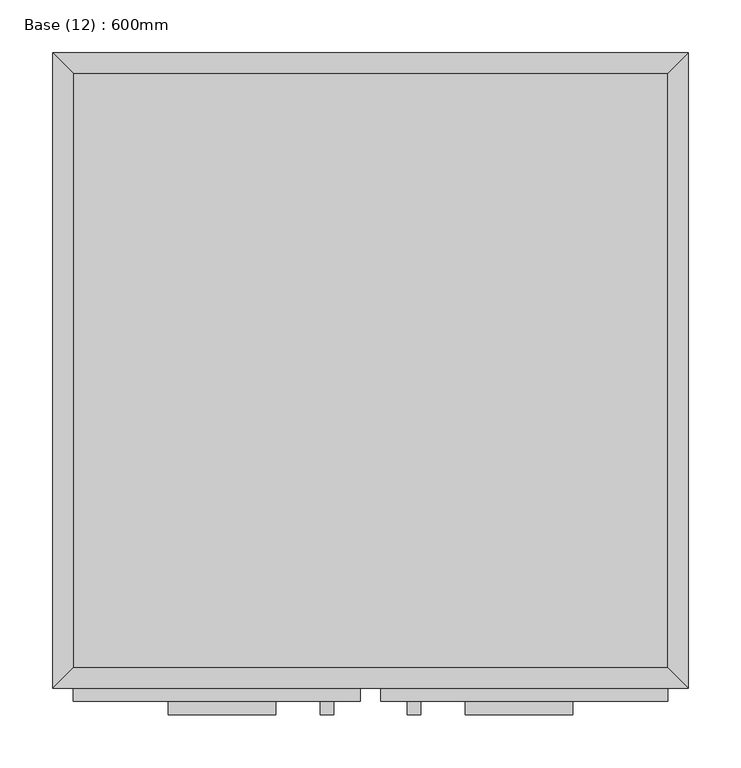
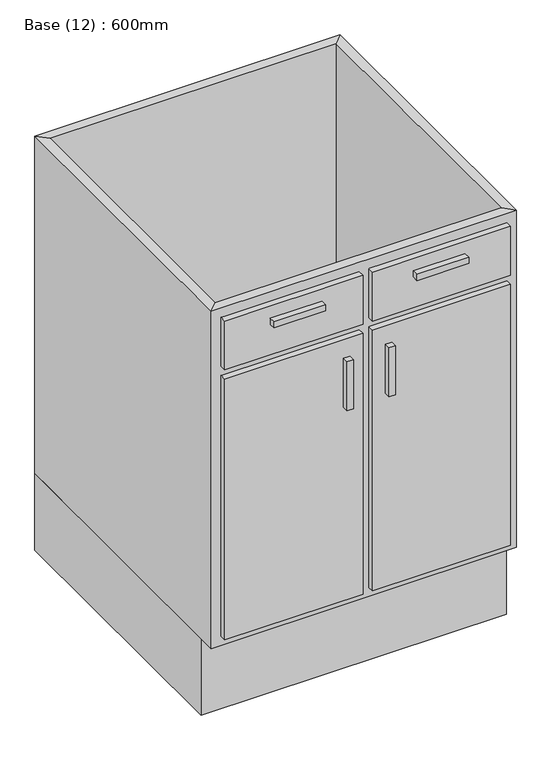
"""IFC4 building model written with IfcOpenShell, lengths in millimetres: furniture geometry, Base (12) : 600mm."""

import ifcopenshell
import ifcopenshell.guid

model = None  # the IFC model being written
_history = None  # IfcOwnerHistory: only IFC2X3 demands one
_inside = {}  # id of a spatial element -> (the spatial element, [elements in it])
_under = {}  # id of a project, library or spatial element -> (it, [spatial elements below it])
_declared = {}  # id of a project -> (the project, [libraries it declares])
_typed = {}  # id of a type object -> (the type object, [elements of that type])
_made_of = {}  # id of a material, layer set ... -> (it, [elements and type objects made of it])


def new_model(schema):
    """Start an empty IFC model of exactly this schema.

    Asked for "IFC4X3", IfcOpenShell would pick the latest addendum, in which some entities
    have other attributes; the version numbers below select the first issue.
    IFC2X3 requires an IfcOwnerHistory on every rooted entity: one is made here for all.
    """
    global model, _history
    if schema == "IFC4X3":
        model = ifcopenshell.file(schema_version=(4, 3, 0, 0))
    else:
        model = ifcopenshell.file(schema=schema)
    _inside.clear()
    _under.clear()
    _declared.clear()
    _typed.clear()
    _made_of.clear()
    _history = None
    if model.schema == "IFC2X3":
        org = make("IfcOrganization", Name="unknown")
        user = make(
            "IfcPersonAndOrganization",
            ThePerson=make("IfcPerson", FamilyName="unknown"),
            TheOrganization=org,
        )
        app = make(
            "IfcApplication",
            ApplicationDeveloper=org,
            Version="unknown",
            ApplicationFullName="unknown",
            ApplicationIdentifier="unknown",
        )
        _history = make(
            "IfcOwnerHistory",
            OwningUser=user,
            OwningApplication=app,
            ChangeAction="ADDED",
            CreationDate=0,
        )
    return model


def make(cls, **values):
    """One entity of the class cls with the attributes given. An attribute that is None is left unset."""
    return model.create_entity(
        cls, **{name: value for name, value in values.items() if value is not None}
    )


def rooted(cls, **values):
    """An entity with a GlobalId (a new one), such as an element, a storey or a relation."""
    return make(cls, GlobalId=ifcopenshell.guid.new(), OwnerHistory=_history, **values)


def si_unit(unit_type, name, prefix=None):
    """IfcSIUnit, for example si_unit("LENGTHUNIT", "METRE", prefix="MILLI")."""
    return make("IfcSIUnit", UnitType=unit_type, Prefix=prefix, Name=name)


def assignment(units):
    """IfcUnitAssignment: the units of a project."""
    return None if units is None else make("IfcUnitAssignment", Units=units)


def point(xyz):
    """IfcCartesianPoint."""
    return None if xyz is None else make("IfcCartesianPoint", Coordinates=xyz)


def direction(xyz):
    """IfcDirection."""
    return None if xyz is None else make("IfcDirection", DirectionRatios=xyz)


def frame(location, z_axis=None, x_axis=None):
    """IfcAxis2Placement3D, a coordinate frame: its origin and axes. An axis left out is left unset."""
    return make(
        "IfcAxis2Placement3D",
        Location=point(location),
        Axis=direction(z_axis),
        RefDirection=direction(x_axis),
    )


def origin():
    """The frame at (0, 0, 0) with its axes left unset."""
    return frame((0.0, 0.0, 0.0))


def origin_with_axes():
    """The frame at (0, 0, 0) with the z axis (0, 0, 1) and the x axis (1, 0, 0) written out."""
    return frame((0.0, 0.0, 0.0), z_axis=(0.0, 0.0, 1.0), x_axis=(1.0, 0.0, 0.0))


def place(relative_to, where):
    """IfcLocalPlacement: puts the frame where relative to a parent placement (None: the world)."""
    return make(
        "IfcLocalPlacement", PlacementRelTo=relative_to, RelativePlacement=where
    )


def context(
    kind, dimensions, precision=None, world=None, true_north=None, identifier=None
):
    """IfcGeometricRepresentationContext, for example the 3D "Model" context."""
    return make(
        "IfcGeometricRepresentationContext",
        ContextIdentifier=identifier,
        ContextType=kind,
        CoordinateSpaceDimension=dimensions,
        Precision=precision,
        WorldCoordinateSystem=world,
        TrueNorth=true_north,
    )


def project(units=None, contexts=None):
    """IfcProject with its units and contexts."""
    return rooted(
        "IfcProject",
        Name="project",
        RepresentationContexts=contexts,
        UnitsInContext=assignment(units),
    )


def spatial(cls, under=None, at=None, **own):
    """A site, building, storey or space (cls), placed at a placement, below another one or the project."""
    s = rooted(cls, ObjectPlacement=at, **own)
    if under is not None:
        _under.setdefault(under.id(), (under, []))[1].append(s)
    return s


def polyline(points):
    """IfcPolyline through the points."""
    return make("IfcPolyline", Points=[point(p) for p in points])


def outline(outer, holes=None, kind="AREA"):
    """IfcArbitraryClosedProfileDef: a profile drawn as a closed curve; with holes, ...WithVoids."""
    if holes is None:
        return make("IfcArbitraryClosedProfileDef", ProfileType=kind, OuterCurve=outer)
    return make(
        "IfcArbitraryProfileDefWithVoids",
        ProfileType=kind,
        OuterCurve=outer,
        InnerCurves=holes,
    )


def extrude(swept, where, along, depth):
    """IfcExtrudedAreaSolid: the profile swept, set in the frame where, extruded along a direction by depth."""
    return make(
        "IfcExtrudedAreaSolid",
        SweptArea=swept,
        Position=where,
        ExtrudedDirection=direction(along),
        Depth=depth,
    )


def faces_of(points, faces, orient=None, outer=None):
    """IfcFace entities. A face is a list of loops; a loop is a list of indices into points, from 0.

    orient and outer hold one flag for each loop. By default every Orientation is true, the
    first loop of a face is its IfcFaceOuterBound and the others are IfcFaceBound.
    """
    made = []
    for i, loops in enumerate(faces):
        bounds = []
        for j, loop in enumerate(loops):
            is_outer = j == 0 if outer is None else outer[i][j]
            bounds.append(
                make(
                    "IfcFaceOuterBound" if is_outer else "IfcFaceBound",
                    Bound=make("IfcPolyLoop", Polygon=[points[k] for k in loop]),
                    Orientation=True if orient is None else orient[i][j],
                )
            )
        made.append(make("IfcFace", Bounds=bounds))
    return made


def faceted_brep(points, faces, orient=None, outer=None, voids=None):
    """IfcFacetedBrep: a solid bounded by flat faces; with voids (closed shells), ...WithVoids."""
    shared = [point(p) for p in points]
    hull = make("IfcClosedShell", CfsFaces=faces_of(shared, faces, orient, outer))
    if voids is None:
        return make("IfcFacetedBrep", Outer=hull)
    return make(
        "IfcFacetedBrepWithVoids",
        Outer=hull,
        Voids=[
            make(cls, CfsFaces=faces_of(shared, fs, o, b)) for cls, fs, o, b in voids
        ],
    )


def shape(context_of_items, identifier, shape_type, items):
    """IfcShapeRepresentation: the items that make up one representation, for example the "Body"."""
    return make(
        "IfcShapeRepresentation",
        ContextOfItems=context_of_items,
        RepresentationIdentifier=identifier,
        RepresentationType=shape_type,
        Items=items,
    )


def source(mapping_origin, context_of_items, identifier, shape_type, items):
    """IfcRepresentationMap: a shape defined once, which mapped items show again and again."""
    return make(
        "IfcRepresentationMap",
        MappingOrigin=mapping_origin,
        MappedRepresentation=shape(context_of_items, identifier, shape_type, items),
    )


def transform(
    local_origin,
    x_axis=None,
    y_axis=None,
    z_axis=None,
    scale=None,
    scale2=None,
    scale3=None,
    uniform=True,
):
    """IfcCartesianTransformationOperator3D, or its non-uniform kind. x_axis, y_axis, z_axis: its Axis1, 2, 3."""
    if uniform:
        return make(
            "IfcCartesianTransformationOperator3D",
            Axis1=direction(x_axis),
            Axis2=direction(y_axis),
            LocalOrigin=point(local_origin),
            Scale=scale,
            Axis3=direction(z_axis),
        )
    return make(
        "IfcCartesianTransformationOperator3DnonUniform",
        Axis1=direction(x_axis),
        Axis2=direction(y_axis),
        LocalOrigin=point(local_origin),
        Scale=scale,
        Axis3=direction(z_axis),
        Scale2=scale2,
        Scale3=scale3,
    )


def mapped(mapping_source, mapping_target):
    """IfcMappedItem: shows the shape of a source again, moved by a transform."""
    return make(
        "IfcMappedItem", MappingSource=mapping_source, MappingTarget=mapping_target
    )


def made_of(thing, what):
    """Note that an element or type object is made of a material, layer set ...; save() writes the relation."""
    if what is not None:
        _made_of.setdefault(what.id(), (what, []))[1].append(thing)
    return thing


def element(
    cls,
    number,
    at=None,
    inside=None,
    cuts=None,
    type_object=None,
    material=None,
    context=None,
    identifier="Body",
    shape_type=None,
    held_by="IfcProductDefinitionShape",
    body=None,
    shapes=None,
    **own,
):
    """One element of the class cls, such as IfcWall. Its Tag is "e" and its number.

    at: its placement. inside: the storey or other place that contains it. cuts: it is an
    opening in that element (IfcRelVoidsElement). A single representation is given by context,
    identifier, shape_type and body (its items); several are given by shapes. held_by: the class
    of the entity that holds the representations. save() writes the other relations.
    """
    e = rooted(cls, Tag="e%d" % number, ObjectPlacement=at, **own)
    if body is not None:
        shapes = [shape(context, identifier, shape_type, body)]
    if shapes is not None:
        e.Representation = make(held_by, Representations=shapes)
    if inside is not None:
        _inside.setdefault(inside.id(), (inside, []))[1].append(e)
    if cuts is not None:
        rooted(
            "IfcRelVoidsElement", RelatingBuildingElement=cuts, RelatedOpeningElement=e
        )
    if type_object is not None:
        _typed.setdefault(type_object.id(), (type_object, []))[1].append(e)
    return made_of(e, material)


def aggregate(whole, parts):
    """IfcRelAggregates: a whole, such as a stair, and the parts it consists of."""
    return rooted("IfcRelAggregates", RelatingObject=whole, RelatedObjects=parts)


def save(model, path):
    """Write the relations noted so far, then the file.

    IfcRelAggregates (storeys below a building ...), IfcRelContainedInSpatialStructure (elements
    in a storey), IfcRelDefinesByType, IfcRelAssociatesMaterial and IfcRelDeclares: one each for
    every whole, place, type object, material and project.
    """
    for whole, parts in _under.values():
        aggregate(whole, parts)
    for where, things in _inside.values():
        rooted(
            "IfcRelContainedInSpatialStructure",
            RelatedElements=things,
            RelatingStructure=where,
        )
    for kind, things in _typed.values():
        rooted("IfcRelDefinesByType", RelatedObjects=things, RelatingType=kind)
    for what, things in _made_of.values():
        rooted("IfcRelAssociatesMaterial", RelatedObjects=things, RelatingMaterial=what)
    for by, libraries in _declared.values():
        rooted("IfcRelDeclares", RelatingContext=by, RelatedDefinitions=libraries)
    model.write(path)


def base_12_600mm_9f03d81e(model_context):
    return source(origin(), model_context, "Body", "SolidModel", [
        extrude(outline(polyline([(299.6877049, -19.05), (299.6877049, -580.95), (-262.2122951, -580.95), (-262.2122951, -19.05), (299.6877049, -19.05)])), frame((0.0, 0.0, 160.0), z_axis=(0.0, 0.0, 1.0), x_axis=(1.0, 0.0, 0.0)), (0.0, 0.0, 1.0), 19.05),
        faceted_brep([(299.6877049, -580.95, 860.0), (299.6877049, -580.95, 160.0), (-262.2122951, -580.95, 160.0), (-262.2122951, -580.95, 860.0), (318.7377049, -600.0, 860.0), (-281.2622951, -600.0, 860.0), (318.7377049, -600.0, 160.0), (-281.2622951, -600.0, 160.0), (-262.2122951, -19.05, 160.0), (-262.2122951, -19.05, 860.0), (-281.2622951, 0.0, 860.0), (-281.2622951, 0.0, 160.0), (299.6877049, -19.05, 160.0), (299.6877049, -19.05, 860.0), (318.7377049, 0.0, 860.0), (318.7377049, 0.0, 160.0)], [[[0, 1, 2, 3]], [[4, 0, 3, 5]], [[6, 4, 5, 7]], [[1, 6, 7, 2]], [[3, 2, 8, 9]], [[5, 3, 9, 10]], [[7, 5, 10, 11]], [[2, 7, 11, 8]], [[9, 8, 12, 13]], [[10, 9, 13, 14]], [[11, 10, 14, 15]], [[8, 11, 15, 12]], [[13, 12, 1, 0]], [[14, 13, 0, 4]], [[15, 14, 4, 6]], [[12, 15, 6, 1]]]),
        extrude(outline(polyline([(318.7377049, 0.0), (318.7377049, -565.0), (-281.2622951, -565.0), (-281.2622951, 0.0), (318.7377049, 0.0)])), origin_with_axes(), (0.0, 0.0, 1.0), 160.0),
        extrude(outline(polyline([(-70.9372951, -625.4), (-172.5372951, -625.4), (-172.5372951, -612.7), (-70.9372951, -612.7), (-70.9372951, -625.4)])), frame((0.0, 0.0, 802.85), z_axis=(0.0, 0.0, 1.0), x_axis=(1.0, 0.0, 0.0)), (0.0, 0.0, 1.0), 12.7),
        extrude(outline(polyline([(210.0127049, -625.4), (108.4127049, -625.4), (108.4127049, -612.7), (210.0127049, -612.7), (210.0127049, -625.4)])), frame((0.0, 0.0, 802.85), z_axis=(0.0, 0.0, 1.0), x_axis=(1.0, 0.0, 0.0)), (0.0, 0.0, 1.0), 12.7),
        extrude(outline(polyline([(-16.1872951, -625.4), (-28.8872951, -625.4), (-28.8872951, -612.7), (-16.1872951, -612.7), (-16.1872951, -625.4)])), frame((0.0, 0.0, 580.6), z_axis=(0.0, 0.0, 1.0), x_axis=(1.0, 0.0, 0.0)), (0.0, 0.0, 1.0), 101.6),
        extrude(outline(polyline([(66.3627049, -625.4), (53.6627049, -625.4), (53.6627049, -612.7), (66.3627049, -612.7), (66.3627049, -625.4)])), frame((0.0, 0.0, 580.6), z_axis=(0.0, 0.0, 1.0), x_axis=(1.0, 0.0, 0.0)), (0.0, 0.0, 1.0), 101.6),
        extrude(outline(polyline([(9.2127049, -612.7), (-262.2122951, -612.7), (-262.2122951, -600.0), (9.2127049, -600.0), (9.2127049, -612.7)])), frame((0.0, 0.0, 739.35), z_axis=(0.0, 0.0, 1.0), x_axis=(1.0, 0.0, 0.0)), (0.0, 0.0, 1.0), 101.6),
        extrude(outline(polyline([(299.6877049, -612.7), (28.2627049, -612.7), (28.2627049, -600.0), (299.6877049, -600.0), (299.6877049, -612.7)])), frame((0.0, 0.0, 739.35), z_axis=(0.0, 0.0, 1.0), x_axis=(1.0, 0.0, 0.0)), (0.0, 0.0, 1.0), 101.6),
        extrude(outline(polyline([(9.2127049, -612.7), (-262.2122951, -612.7), (-262.2122951, -600.0), (9.2127049, -600.0), (9.2127049, -612.7)])), frame((0.0, 0.0, 179.05), z_axis=(0.0, 0.0, 1.0), x_axis=(1.0, 0.0, 0.0)), (0.0, 0.0, 1.0), 541.25),
        extrude(outline(polyline([(299.6877049, -612.7), (28.2627049, -612.7), (28.2627049, -600.0), (299.6877049, -600.0), (299.6877049, -612.7)])), frame((0.0, 0.0, 179.05), z_axis=(0.0, 0.0, 1.0), x_axis=(1.0, 0.0, 0.0)), (0.0, 0.0, 1.0), 541.25),
    ])


if __name__ == "__main__":
    model = new_model("IFC4")
    model_context = context("Model", 3, world=origin())
    ifc_project = project(units=[si_unit("LENGTHUNIT", "METRE", prefix="MILLI")], contexts=[model_context])
    site = spatial("IfcSite", under=ifc_project)
    building = spatial("IfcBuilding", under=site)
    placement = place(None, origin())
    base_12_600mm_shape = base_12_600mm_9f03d81e(model_context)
    element("IfcFurniture", 1, ObjectType="Base (12) : 600mm", at=placement, inside=building, context=model_context, shape_type="MappedRepresentation", body=[
        mapped(base_12_600mm_shape, transform((0.0, 0.0, 0.0), x_axis=(1.0, 0.0, 0.0), y_axis=(0.0, 1.0, 0.0), z_axis=(0.0, 0.0, 1.0))),
    ])
    save(model, "model.ifc")

# Revit data of these elements
# Type "Base (12) : 600mm"
#   Keynote = "N10"
#   Depth = 600 mm
#   Height = 860 mm
#   Plinth Depth = 35 mm
#   Plinth Height = 160 mm
#   Width = 600 mm
#   Material Cabinet = Cabinets
#   Material Door/Drawer = Cabinets
#   Material Handle = Cabinets - Handles
# Element 1 (IfcFurniture, "Base (12) : 600mm")
#   Materials on its faces: "Cabinets", "Cabinets - Handles"
# Materials
#   "Cabinets": class "Miscellaneous", colour RGB 249 249 249, transparency 0
#   "Cabinets - Handles": class "Metal", colour RGB 57 57 57, transparency 0
